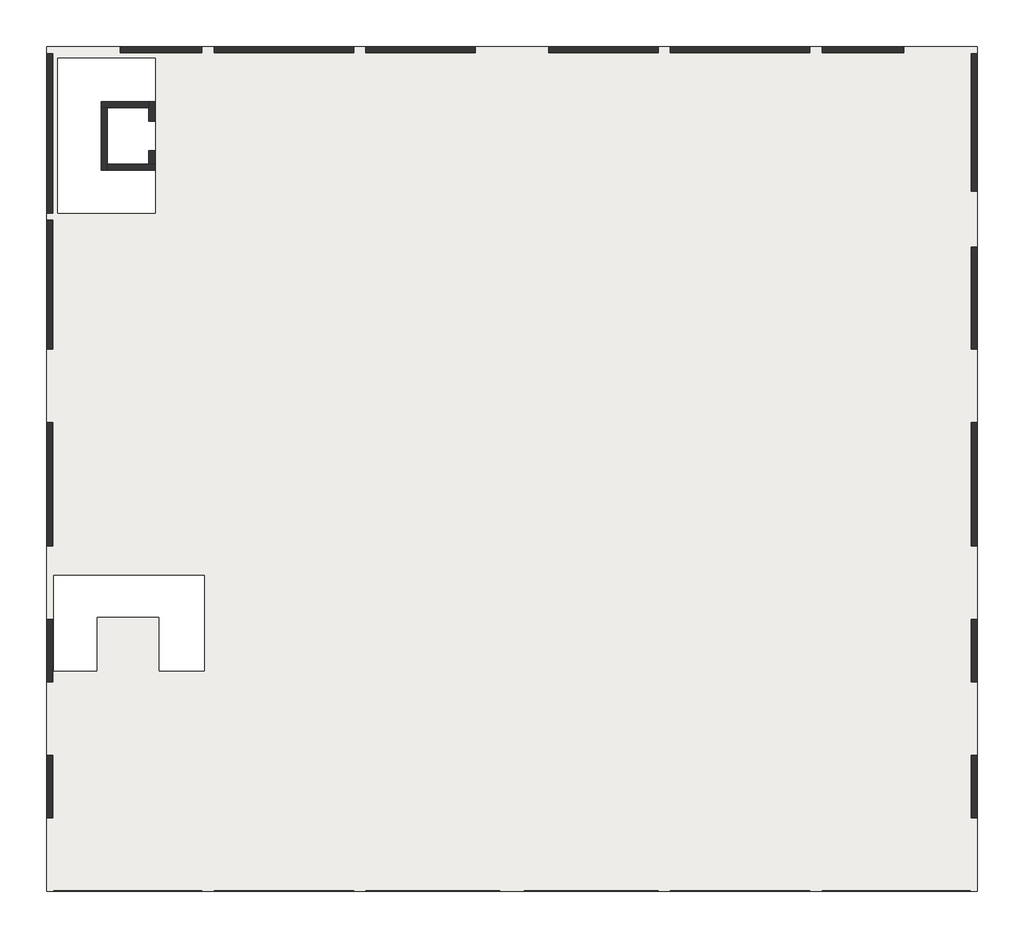
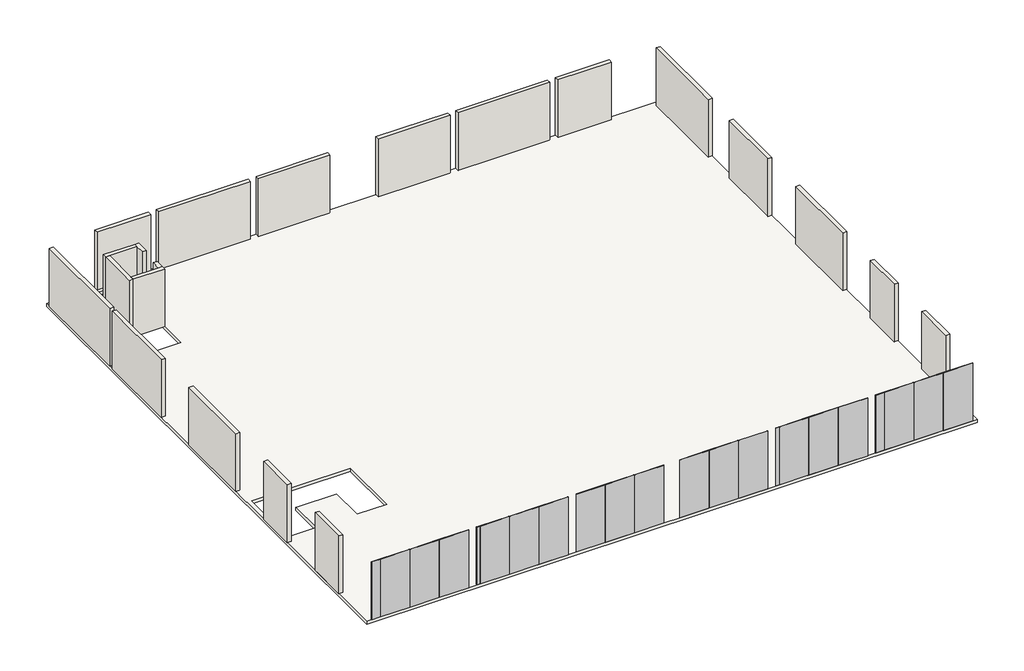
# One storey: 22 plates, 21 walls, 1 slab.
"""IFC4 building model written with IfcOpenShell, lengths in millimetres."""

import ifcopenshell
import ifcopenshell.guid

model = None  # the IFC model being written
_history = None  # IfcOwnerHistory: only IFC2X3 demands one
_inside = {}  # id of a spatial element -> (the spatial element, [elements in it])
_under = {}  # id of a project, library or spatial element -> (it, [spatial elements below it])
_declared = {}  # id of a project -> (the project, [libraries it declares])
_typed = {}  # id of a type object -> (the type object, [elements of that type])
_made_of = {}  # id of a material, layer set ... -> (it, [elements and type objects made of it])


def new_model(schema):
    """Start an empty IFC model of exactly this schema.

    Asked for "IFC4X3", IfcOpenShell would pick the latest addendum, in which some entities
    have other attributes; the version numbers below select the first issue.
    IFC2X3 requires an IfcOwnerHistory on every rooted entity: one is made here for all.
    """
    global model, _history
    if schema == "IFC4X3":
        model = ifcopenshell.file(schema_version=(4, 3, 0, 0))
    else:
        model = ifcopenshell.file(schema=schema)
    _inside.clear()
    _under.clear()
    _declared.clear()
    _typed.clear()
    _made_of.clear()
    _history = None
    if model.schema == "IFC2X3":
        org = make("IfcOrganization", Name="unknown")
        user = make(
            "IfcPersonAndOrganization",
            ThePerson=make("IfcPerson", FamilyName="unknown"),
            TheOrganization=org,
        )
        app = make(
            "IfcApplication",
            ApplicationDeveloper=org,
            Version="unknown",
            ApplicationFullName="unknown",
            ApplicationIdentifier="unknown",
        )
        _history = make(
            "IfcOwnerHistory",
            OwningUser=user,
            OwningApplication=app,
            ChangeAction="ADDED",
            CreationDate=0,
        )
    return model


def make(cls, **values):
    """One entity of the class cls with the attributes given. An attribute that is None is left unset."""
    return model.create_entity(
        cls, **{name: value for name, value in values.items() if value is not None}
    )


def rooted(cls, **values):
    """An entity with a GlobalId (a new one), such as an element, a storey or a relation."""
    return make(cls, GlobalId=ifcopenshell.guid.new(), OwnerHistory=_history, **values)


def si_unit(unit_type, name, prefix=None):
    """IfcSIUnit, for example si_unit("LENGTHUNIT", "METRE", prefix="MILLI")."""
    return make("IfcSIUnit", UnitType=unit_type, Prefix=prefix, Name=name)


def assignment(units):
    """IfcUnitAssignment: the units of a project."""
    return None if units is None else make("IfcUnitAssignment", Units=units)


def point(xyz):
    """IfcCartesianPoint."""
    return None if xyz is None else make("IfcCartesianPoint", Coordinates=xyz)


def direction(xyz):
    """IfcDirection."""
    return None if xyz is None else make("IfcDirection", DirectionRatios=xyz)


def frame(location, z_axis=None, x_axis=None):
    """IfcAxis2Placement3D, a coordinate frame: its origin and axes. An axis left out is left unset."""
    return make(
        "IfcAxis2Placement3D",
        Location=point(location),
        Axis=direction(z_axis),
        RefDirection=direction(x_axis),
    )


def origin():
    """The frame at (0, 0, 0) with its axes left unset."""
    return frame((0.0, 0.0, 0.0))


def origin_with_axes():
    """The frame at (0, 0, 0) with the z axis (0, 0, 1) and the x axis (1, 0, 0) written out."""
    return frame((0.0, 0.0, 0.0), z_axis=(0.0, 0.0, 1.0), x_axis=(1.0, 0.0, 0.0))


def place(relative_to, where):
    """IfcLocalPlacement: puts the frame where relative to a parent placement (None: the world)."""
    return make(
        "IfcLocalPlacement", PlacementRelTo=relative_to, RelativePlacement=where
    )


def context(
    kind, dimensions, precision=None, world=None, true_north=None, identifier=None
):
    """IfcGeometricRepresentationContext, for example the 3D "Model" context."""
    return make(
        "IfcGeometricRepresentationContext",
        ContextIdentifier=identifier,
        ContextType=kind,
        CoordinateSpaceDimension=dimensions,
        Precision=precision,
        WorldCoordinateSystem=world,
        TrueNorth=true_north,
    )


def project(units=None, contexts=None):
    """IfcProject with its units and contexts."""
    return rooted(
        "IfcProject",
        Name="project",
        RepresentationContexts=contexts,
        UnitsInContext=assignment(units),
    )


def spatial(cls, under=None, at=None, **own):
    """A site, building, storey or space (cls), placed at a placement, below another one or the project."""
    s = rooted(cls, ObjectPlacement=at, **own)
    if under is not None:
        _under.setdefault(under.id(), (under, []))[1].append(s)
    return s


def polyline(points):
    """IfcPolyline through the points."""
    return make("IfcPolyline", Points=[point(p) for p in points])


def outline(outer, holes=None, kind="AREA"):
    """IfcArbitraryClosedProfileDef: a profile drawn as a closed curve; with holes, ...WithVoids."""
    if holes is None:
        return make("IfcArbitraryClosedProfileDef", ProfileType=kind, OuterCurve=outer)
    return make(
        "IfcArbitraryProfileDefWithVoids",
        ProfileType=kind,
        OuterCurve=outer,
        InnerCurves=holes,
    )


def extrude(swept, where, along, depth):
    """IfcExtrudedAreaSolid: the profile swept, set in the frame where, extruded along a direction by depth."""
    return make(
        "IfcExtrudedAreaSolid",
        SweptArea=swept,
        Position=where,
        ExtrudedDirection=direction(along),
        Depth=depth,
    )


def faces_of(points, faces, orient=None, outer=None):
    """IfcFace entities. A face is a list of loops; a loop is a list of indices into points, from 0.

    orient and outer hold one flag for each loop. By default every Orientation is true, the
    first loop of a face is its IfcFaceOuterBound and the others are IfcFaceBound.
    """
    made = []
    for i, loops in enumerate(faces):
        bounds = []
        for j, loop in enumerate(loops):
            is_outer = j == 0 if outer is None else outer[i][j]
            bounds.append(
                make(
                    "IfcFaceOuterBound" if is_outer else "IfcFaceBound",
                    Bound=make("IfcPolyLoop", Polygon=[points[k] for k in loop]),
                    Orientation=True if orient is None else orient[i][j],
                )
            )
        made.append(make("IfcFace", Bounds=bounds))
    return made


def faceted_brep(points, faces, orient=None, outer=None, voids=None):
    """IfcFacetedBrep: a solid bounded by flat faces; with voids (closed shells), ...WithVoids."""
    shared = [point(p) for p in points]
    hull = make("IfcClosedShell", CfsFaces=faces_of(shared, faces, orient, outer))
    if voids is None:
        return make("IfcFacetedBrep", Outer=hull)
    return make(
        "IfcFacetedBrepWithVoids",
        Outer=hull,
        Voids=[
            make(cls, CfsFaces=faces_of(shared, fs, o, b)) for cls, fs, o, b in voids
        ],
    )


def shape(context_of_items, identifier, shape_type, items):
    """IfcShapeRepresentation: the items that make up one representation, for example the "Body"."""
    return make(
        "IfcShapeRepresentation",
        ContextOfItems=context_of_items,
        RepresentationIdentifier=identifier,
        RepresentationType=shape_type,
        Items=items,
    )


def source(mapping_origin, context_of_items, identifier, shape_type, items):
    """IfcRepresentationMap: a shape defined once, which mapped items show again and again."""
    return make(
        "IfcRepresentationMap",
        MappingOrigin=mapping_origin,
        MappedRepresentation=shape(context_of_items, identifier, shape_type, items),
    )


def transform(
    local_origin,
    x_axis=None,
    y_axis=None,
    z_axis=None,
    scale=None,
    scale2=None,
    scale3=None,
    uniform=True,
):
    """IfcCartesianTransformationOperator3D, or its non-uniform kind. x_axis, y_axis, z_axis: its Axis1, 2, 3."""
    if uniform:
        return make(
            "IfcCartesianTransformationOperator3D",
            Axis1=direction(x_axis),
            Axis2=direction(y_axis),
            LocalOrigin=point(local_origin),
            Scale=scale,
            Axis3=direction(z_axis),
        )
    return make(
        "IfcCartesianTransformationOperator3DnonUniform",
        Axis1=direction(x_axis),
        Axis2=direction(y_axis),
        LocalOrigin=point(local_origin),
        Scale=scale,
        Axis3=direction(z_axis),
        Scale2=scale2,
        Scale3=scale3,
    )


def mapped(mapping_source, mapping_target):
    """IfcMappedItem: shows the shape of a source again, moved by a transform."""
    return make(
        "IfcMappedItem", MappingSource=mapping_source, MappingTarget=mapping_target
    )


def made_of(thing, what):
    """Note that an element or type object is made of a material, layer set ...; save() writes the relation."""
    if what is not None:
        _made_of.setdefault(what.id(), (what, []))[1].append(thing)
    return thing


def element(
    cls,
    number,
    at=None,
    inside=None,
    cuts=None,
    type_object=None,
    material=None,
    context=None,
    identifier="Body",
    shape_type=None,
    held_by="IfcProductDefinitionShape",
    body=None,
    shapes=None,
    **own,
):
    """One element of the class cls, such as IfcWall. Its Tag is "e" and its number.

    at: its placement. inside: the storey or other place that contains it. cuts: it is an
    opening in that element (IfcRelVoidsElement). A single representation is given by context,
    identifier, shape_type and body (its items); several are given by shapes. held_by: the class
    of the entity that holds the representations. save() writes the other relations.
    """
    e = rooted(cls, Tag="e%d" % number, ObjectPlacement=at, **own)
    if body is not None:
        shapes = [shape(context, identifier, shape_type, body)]
    if shapes is not None:
        e.Representation = make(held_by, Representations=shapes)
    if inside is not None:
        _inside.setdefault(inside.id(), (inside, []))[1].append(e)
    if cuts is not None:
        rooted(
            "IfcRelVoidsElement", RelatingBuildingElement=cuts, RelatedOpeningElement=e
        )
    if type_object is not None:
        _typed.setdefault(type_object.id(), (type_object, []))[1].append(e)
    return made_of(e, material)


def aggregate(whole, parts):
    """IfcRelAggregates: a whole, such as a stair, and the parts it consists of."""
    return rooted("IfcRelAggregates", RelatingObject=whole, RelatedObjects=parts)


def save(model, path):
    """Write the relations noted so far, then the file.

    IfcRelAggregates (storeys below a building ...), IfcRelContainedInSpatialStructure (elements
    in a storey), IfcRelDefinesByType, IfcRelAssociatesMaterial and IfcRelDeclares: one each for
    every whole, place, type object, material and project.
    """
    for whole, parts in _under.values():
        aggregate(whole, parts)
    for where, things in _inside.values():
        rooted(
            "IfcRelContainedInSpatialStructure",
            RelatedElements=things,
            RelatingStructure=where,
        )
    for kind, things in _typed.values():
        rooted("IfcRelDefinesByType", RelatedObjects=things, RelatingType=kind)
    for what, things in _made_of.values():
        rooted("IfcRelAssociatesMaterial", RelatedObjects=things, RelatingMaterial=what)
    for by, libraries in _declared.values():
        rooted("IfcRelDeclares", RelatingContext=by, RelatedDefinitions=libraries)
    model.write(path)


def system_panel_glazed_0b61e5af(model_context):
    return source(origin(), model_context, "Body", "SweptSolid", [
        extrude(outline(polyline([(915.0000002, 24.5), (-915.0000002, 24.5), (-915.0000002, 49.5), (915.0000002, 49.5), (915.0000002, 24.5)])), origin_with_axes(), (0.0, 0.0, 1.0), 3800.0),
    ])


def system_panel_glazed_e3bcbcf3(model_context):
    return source(origin(), model_context, "Body", "SweptSolid", [
        extrude(outline(polyline([(274.9999998, 24.5), (-274.9999998, 24.5), (-274.9999998, 49.5), (274.9999998, 49.5), (274.9999998, 24.5)])), origin_with_axes(), (0.0, 0.0, 1.0), 3800.0),
    ])


def system_panel_glazed_31375f6b(model_context):
    return source(origin(), model_context, "Body", "SweptSolid", [
        extrude(outline(polyline([(104.9999998, 24.5), (-104.9999998, 24.5), (-104.9999998, 49.5), (104.9999998, 49.5), (104.9999998, 24.5)])), origin_with_axes(), (0.0, 0.0, 1.0), 3800.0),
    ])


def system_panel_glazed_aacaf49b(model_context):
    return source(origin(), model_context, "Body", "SweptSolid", [
        extrude(outline(polyline([(904.9999998, 24.5), (-904.9999998, 24.5), (-904.9999998, 49.5), (904.9999998, 49.5), (904.9999998, 24.5)])), origin_with_axes(), (0.0, 0.0, 1.0), 3800.0),
    ])


def system_panel_glazed_e1325fc6(model_context):
    return source(origin(), model_context, "Body", "SweptSolid", [
        extrude(outline(polyline([(894.9999998, 24.5), (-894.9999998, 24.5), (-894.9999998, 49.5), (894.9999998, 49.5), (894.9999998, 24.5)])), origin_with_axes(), (0.0, 0.0, 1.0), 3800.0),
    ])


model = new_model("IFC4")

# Units and contexts
model_context = context("Model", 3, world=origin())
ifc_project = project(units=[si_unit("LENGTHUNIT", "METRE", prefix="MILLI")], contexts=[model_context])

# Site, building, storey
site = spatial("IfcSite", under=ifc_project)
building = spatial("IfcBuilding", under=site)
storey = spatial("IfcBuildingStorey", under=building, Name="Perdhesa", Elevation=0.0)

# Plates
placement = place(None, origin())
system_panel_glazed_shape = system_panel_glazed_0b61e5af(model_context)
element("IfcPlate", 1, ObjectType="System Panel : Glazed", at=placement, inside=storey, context=model_context, shape_type="MappedRepresentation", body=[
    mapped(system_panel_glazed_shape, transform((18910.5819109, -16669.9481037, 0.0), x_axis=(-1.0, 0.0, 0.0), y_axis=(0.0, -1.0, 0.0), z_axis=(0.0, 0.0, 1.0))),
])
element("IfcPlate", 2, ObjectType="System Panel : Glazed", at=placement, inside=storey, context=model_context, shape_type="MappedRepresentation", body=[
    mapped(system_panel_glazed_shape, transform((17080.5819107, -16669.9481037, 0.0), x_axis=(-1.0, 0.0, 0.0), y_axis=(0.0, -1.0, 0.0), z_axis=(0.0, 0.0, 1.0))),
])
element("IfcPlate", 3, ObjectType="System Panel : Glazed", at=placement, inside=storey, context=model_context, shape_type="MappedRepresentation", body=[
    mapped(system_panel_glazed_shape, transform((15250.5819107, -16669.9481037, 0.0), x_axis=(-1.0, 0.0, 0.0), y_axis=(0.0, -1.0, 0.0), z_axis=(0.0, 0.0, 1.0))),
])
element("IfcPlate", 4, ObjectType="System Panel : Glazed", at=placement, inside=storey, context=model_context, shape_type="MappedRepresentation", body=[
    mapped(system_panel_glazed_shape, transform((12370.5819109, -16669.9481037, 0.0), x_axis=(-1.0, 0.0, 0.0), y_axis=(0.0, -1.0, 0.0), z_axis=(0.0, 0.0, 1.0))),
])
element("IfcPlate", 5, ObjectType="System Panel : Glazed", at=placement, inside=storey, context=model_context, shape_type="MappedRepresentation", body=[
    mapped(system_panel_glazed_shape, transform((10540.5819107, -16669.9481037, 0.0), x_axis=(-1.0, 0.0, 0.0), y_axis=(0.0, -1.0, 0.0), z_axis=(0.0, 0.0, 1.0))),
])
element("IfcPlate", 6, ObjectType="System Panel : Glazed", at=placement, inside=storey, context=model_context, shape_type="MappedRepresentation", body=[
    mapped(system_panel_glazed_shape, transform((8710.5819107, -16669.9481037, 0.0), x_axis=(-1.0, 0.0, 0.0), y_axis=(0.0, -1.0, 0.0), z_axis=(0.0, 0.0, 1.0))),
])
element("IfcPlate", 7, ObjectType="System Panel : Glazed", at=placement, inside=storey, context=model_context, shape_type="MappedRepresentation", body=[
    mapped(system_panel_glazed_shape, transform((6170.5819109, -16669.9481037, 0.0), x_axis=(-1.0, 0.0, 0.0), y_axis=(0.0, -1.0, 0.0), z_axis=(0.0, 0.0, 1.0))),
])
element("IfcPlate", 8, ObjectType="System Panel : Glazed", at=placement, inside=storey, context=model_context, shape_type="MappedRepresentation", body=[
    mapped(system_panel_glazed_shape, transform((4340.5819107, -16669.9481037, 0.0), x_axis=(-1.0, 0.0, 0.0), y_axis=(0.0, -1.0, 0.0), z_axis=(0.0, 0.0, 1.0))),
])
element("IfcPlate", 9, ObjectType="System Panel : Glazed", at=placement, inside=storey, context=model_context, shape_type="MappedRepresentation", body=[
    mapped(system_panel_glazed_shape, transform((-299.4180891, -16669.9481037, 0.0), x_axis=(-1.0, 0.0, 0.0), y_axis=(0.0, -1.0, 0.0), z_axis=(0.0, 0.0, 1.0))),
])
element("IfcPlate", 10, ObjectType="System Panel : Glazed", at=placement, inside=storey, context=model_context, shape_type="MappedRepresentation", body=[
    mapped(system_panel_glazed_shape, transform((-2129.4180893, -16669.9481037, 0.0), x_axis=(-1.0, 0.0, 0.0), y_axis=(0.0, -1.0, 0.0), z_axis=(0.0, 0.0, 1.0))),
])
element("IfcPlate", 11, ObjectType="System Panel : Glazed", at=placement, inside=storey, context=model_context, shape_type="MappedRepresentation", body=[
    mapped(system_panel_glazed_shape, transform((-6249.4180891, -16669.9481037, 0.0), x_axis=(-1.0, 0.0, 0.0), y_axis=(0.0, -1.0, 0.0), z_axis=(0.0, 0.0, 1.0))),
])
element("IfcPlate", 12, ObjectType="System Panel : Glazed", at=placement, inside=storey, context=model_context, shape_type="MappedRepresentation", body=[
    mapped(system_panel_glazed_shape, transform((-8079.4180893, -16669.9481037, 0.0), x_axis=(-1.0, 0.0, 0.0), y_axis=(0.0, -1.0, 0.0), z_axis=(0.0, 0.0, 1.0))),
])
element("IfcPlate", 13, ObjectType="System Panel : Glazed", at=placement, inside=storey, context=model_context, shape_type="MappedRepresentation", body=[
    mapped(system_panel_glazed_shape, transform((-9909.4180893, -16669.9481037, 0.0), x_axis=(-1.0, 0.0, 0.0), y_axis=(0.0, -1.0, 0.0), z_axis=(0.0, 0.0, 1.0))),
])
element("IfcPlate", 14, ObjectType="System Panel : Glazed", at=placement, inside=storey, context=model_context, shape_type="MappedRepresentation", body=[
    mapped(system_panel_glazed_shape, transform((-12449.4180891, -16669.9481037, 0.0), x_axis=(-1.0, 0.0, 0.0), y_axis=(0.0, -1.0, 0.0), z_axis=(0.0, 0.0, 1.0))),
])
element("IfcPlate", 15, ObjectType="System Panel : Glazed", at=placement, inside=storey, context=model_context, shape_type="MappedRepresentation", body=[
    mapped(system_panel_glazed_shape, transform((-14279.4180893, -16669.9481037, 0.0), x_axis=(-1.0, 0.0, 0.0), y_axis=(0.0, -1.0, 0.0), z_axis=(0.0, 0.0, 1.0))),
])
element("IfcPlate", 16, ObjectType="System Panel : Glazed", at=placement, inside=storey, context=model_context, shape_type="MappedRepresentation", body=[
    mapped(system_panel_glazed_shape, transform((-16109.4180893, -16669.9481037, 0.0), x_axis=(-1.0, 0.0, 0.0), y_axis=(0.0, -1.0, 0.0), z_axis=(0.0, 0.0, 1.0))),
])
system_panel_glazed_2_shape = system_panel_glazed_e3bcbcf3(model_context)
element("IfcPlate", 17, ObjectType="System Panel : Glazed", at=placement, inside=storey, context=model_context, shape_type="MappedRepresentation", body=[
    mapped(system_panel_glazed_2_shape, transform((14060.5819109, -16669.9481037, 0.0), x_axis=(-1.0, 0.0, 0.0), y_axis=(0.0, -1.0, 0.0), z_axis=(0.0, 0.0, 1.0))),
])
element("IfcPlate", 18, ObjectType="System Panel : Glazed", at=placement, inside=storey, context=model_context, shape_type="MappedRepresentation", body=[
    mapped(system_panel_glazed_2_shape, transform((-17299.4180891, -16669.9481037, 0.0), x_axis=(-1.0, 0.0, 0.0), y_axis=(0.0, -1.0, 0.0), z_axis=(0.0, 0.0, 1.0))),
])
system_panel_glazed_3_shape = system_panel_glazed_31375f6b(model_context)
element("IfcPlate", 19, ObjectType="System Panel : Glazed", at=placement, inside=storey, context=model_context, shape_type="MappedRepresentation", body=[
    mapped(system_panel_glazed_3_shape, transform((7690.5819109, -16669.9481037, 0.0), x_axis=(-1.0, 0.0, 0.0), y_axis=(0.0, -1.0, 0.0), z_axis=(0.0, 0.0, 1.0))),
])
element("IfcPlate", 20, ObjectType="System Panel : Glazed", at=placement, inside=storey, context=model_context, shape_type="MappedRepresentation", body=[
    mapped(system_panel_glazed_3_shape, transform((-10929.4180891, -16669.9481037, 0.0), x_axis=(-1.0, 0.0, 0.0), y_axis=(0.0, -1.0, 0.0), z_axis=(0.0, 0.0, 1.0))),
])
system_panel_glazed_4_shape = system_panel_glazed_aacaf49b(model_context)
element("IfcPlate", 21, ObjectType="System Panel : Glazed", at=placement, inside=storey, context=model_context, shape_type="MappedRepresentation", body=[
    mapped(system_panel_glazed_4_shape, transform((2520.5819109, -16669.9481037, 0.0), x_axis=(-1.0, 0.0, 0.0), y_axis=(0.0, -1.0, 0.0), z_axis=(0.0, 0.0, 1.0))),
])
system_panel_glazed_5_shape = system_panel_glazed_e1325fc6(model_context)
element("IfcPlate", 22, ObjectType="System Panel : Glazed", at=placement, inside=storey, context=model_context, shape_type="MappedRepresentation", body=[
    mapped(system_panel_glazed_5_shape, transform((-3939.4180891, -16669.9481037, 0.0), x_axis=(-1.0, 0.0, 0.0), y_axis=(0.0, -1.0, 0.0), z_axis=(0.0, 0.0, 1.0))),
])

# Slab
element("IfcSlab", 23, ObjectType="Generic 20", at=placement, inside=storey, context=model_context, shape_type="SweptSolid", body=[
    extrude(outline(polyline([(20125.581911, 17780.6768963), (20125.581911, -16719.3231037), (-17874.418089, -16719.3231037), (-17874.418089, 17780.6768963), (20125.581911, 17780.6768963)]), holes=[polyline([(-17424.418089, 17310.6768963), (-17424.418089, 10980.6768963), (-13444.418089, 10980.6768963), (-13444.418089, 17310.6768963), (-17424.418089, 17310.6768963)]), polyline([(-15825.6814495, -5518.0731037), (-13265.2814495, -5518.0731037), (-13265.2814495, -7718.0731037), (-11435.2814495, -7718.0731037), (-11435.2814495, -3818.0731037), (-17574.418089, -3818.0731037), (-17574.418089, -7718.0731037), (-15825.6814495, -7718.0731037), (-15825.6814495, -5518.0731037)])]), frame((0.0, 0.0, -200.0), z_axis=(0.0, 0.0, 1.0), x_axis=(1.0, 0.0, 0.0)), (0.0, 0.0, 1.0), 200.0),
])

# Walls
element("IfcWall", 24, ObjectType="lifti", at=placement, inside=storey, context=model_context, shape_type="Brep", body=[
    faceted_brep([(-15644.418089, 15280.6768963, 0.0), (-15394.418089, 15280.6768963, 0.0), (-13694.418089, 15280.6768963, 0.0), (-13694.418089, 15280.6768963, 3800.0), (-15394.418089, 15280.6768963, 3800.0), (-15644.418089, 15280.6768963, 3800.0), (-15644.418089, 15530.6768963, 0.0), (-15644.418089, 15530.6768963, 3800.0), (-13694.418089, 15530.6768963, 3800.0), (-13694.418089, 15530.6768963, 0.0)], [[[0, 1, 2, 3, 4, 5]], [[6, 7, 8, 9]], [[2, 1, 0, 6, 9]], [[5, 4, 3, 8, 7]], [[0, 5, 7, 6]], [[3, 2, 9, 8]]]),
])
element("IfcWall", 25, ObjectType="lifti", at=placement, inside=storey, context=model_context, shape_type="Brep", body=[
    faceted_brep([(-15394.418089, 12730.6768963, 0.0), (-15394.418089, 12980.6768963, 0.0), (-15394.418089, 15280.6768963, 0.0), (-15394.418089, 15280.6768963, 3800.0), (-15394.418089, 12980.6768963, 3800.0), (-15394.418089, 12730.6768963, 3800.0), (-15644.418089, 12730.6768963, 0.0), (-15644.418089, 12730.6768963, 3800.0), (-15644.418089, 15280.6768963, 3800.0), (-15644.418089, 15280.6768963, 0.0)], [[[0, 1, 2, 3, 4, 5]], [[6, 7, 8, 9]], [[2, 1, 0, 6, 9]], [[5, 4, 3, 8, 7]], [[0, 5, 7, 6]], [[3, 2, 9, 8]]]),
])
element("IfcWall", 26, ObjectType="lifti", at=placement, inside=storey, context=model_context, shape_type="Brep", body=[
    faceted_brep([(-13444.418089, 12980.6768963, 0.0), (-13694.418089, 12980.6768963, 0.0), (-15394.418089, 12980.6768963, 0.0), (-15394.418089, 12980.6768963, 3800.0), (-13694.418089, 12980.6768963, 3800.0), (-13444.418089, 12980.6768963, 3800.0), (-13444.418089, 12730.6768963, 0.0), (-13444.418089, 12730.6768963, 3800.0), (-15394.418089, 12730.6768963, 3800.0), (-15394.418089, 12730.6768963, 0.0)], [[[0, 1, 2, 3, 4, 5]], [[6, 7, 8, 9]], [[2, 1, 0, 6, 9]], [[5, 4, 3, 8, 7]], [[0, 5, 7, 6]], [[3, 2, 9, 8]]]),
])
element("IfcWall", 27, ObjectType="lifti", at=placement, inside=storey, context=model_context, shape_type="Brep", body=[
    faceted_brep([(-13694.418089, 15530.6768963, 0.0), (-13694.418089, 15280.6768963, 0.0), (-13694.418089, 14730.6768963, 0.0), (-13694.418089, 14730.6768963, 3800.0), (-13694.418089, 15280.6768963, 3800.0), (-13694.418089, 15530.6768963, 3800.0), (-13444.418089, 15530.6768963, 0.0), (-13444.418089, 15530.6768963, 3800.0), (-13444.418089, 14730.6768963, 3800.0), (-13444.418089, 14730.6768963, 0.0)], [[[0, 1, 2, 3, 4, 5]], [[6, 7, 8, 9]], [[2, 1, 0, 6, 9]], [[3, 2, 9, 8]], [[5, 4, 3, 8, 7]], [[0, 5, 7, 6]]]),
])
element("IfcWall", 28, ObjectType="lifti", at=placement, inside=storey, context=model_context, shape_type="SweptSolid", body=[
    extrude(outline(polyline([(-13694.418089, 12980.6768963), (-13694.418089, 13530.6768963), (-13444.418089, 13530.6768963), (-13444.418089, 12980.6768963), (-13694.418089, 12980.6768963)])), origin_with_axes(), (0.0, 0.0, 1.0), 3800.0),
])
element("IfcWall", 29, ObjectType="Generic - 250", at=placement, inside=storey, context=model_context, shape_type="SweptSolid", body=[
    extrude(outline(polyline([(-17874.418089, 10980.6768963), (-17874.418089, 17480.6768963), (-17624.418089, 17480.6768963), (-17624.418089, 10980.6768963), (-17874.418089, 10980.6768963)])), origin_with_axes(), (0.0, 0.0, 1.0), 3800.0),
])
element("IfcWall", 30, ObjectType="Generic - 250", at=placement, inside=storey, context=model_context, shape_type="SweptSolid", body=[
    extrude(outline(polyline([(-11534.418089, 17530.6768963), (-14874.418089, 17530.6768963), (-14874.418089, 17780.6768963), (-11534.418089, 17780.6768963), (-11534.418089, 17530.6768963)])), origin_with_axes(), (0.0, 0.0, 1.0), 3800.0),
])
element("IfcWall", 31, ObjectType="Generic - 250", at=placement, inside=storey, context=model_context, shape_type="SweptSolid", body=[
    extrude(outline(polyline([(-5334.418089, 17530.6768963), (-11034.418089, 17530.6768963), (-11034.418089, 17780.6768963), (-5334.418089, 17780.6768963), (-5334.418089, 17530.6768963)])), origin_with_axes(), (0.0, 0.0, 1.0), 3800.0),
])
element("IfcWall", 32, ObjectType="Generic - 250", at=placement, inside=storey, context=model_context, shape_type="SweptSolid", body=[
    extrude(outline(polyline([(-384.418089, 17530.6768963), (-4834.418089, 17530.6768963), (-4834.418089, 17780.6768963), (-384.418089, 17780.6768963), (-384.418089, 17530.6768963)])), origin_with_axes(), (0.0, 0.0, 1.0), 3800.0),
])
element("IfcWall", 33, ObjectType="Generic - 250", at=placement, inside=storey, context=model_context, shape_type="SweptSolid", body=[
    extrude(outline(polyline([(7085.581911, 17530.6768963), (2615.581911, 17530.6768963), (2615.581911, 17780.6768963), (7085.581911, 17780.6768963), (7085.581911, 17530.6768963)])), origin_with_axes(), (0.0, 0.0, 1.0), 3800.0),
])
element("IfcWall", 34, ObjectType="Generic - 250", at=placement, inside=storey, context=model_context, shape_type="SweptSolid", body=[
    extrude(outline(polyline([(13285.581911, 17530.6768963), (7585.581911, 17530.6768963), (7585.581911, 17780.6768963), (13285.581911, 17780.6768963), (13285.581911, 17530.6768963)])), origin_with_axes(), (0.0, 0.0, 1.0), 3800.0),
])
element("IfcWall", 35, ObjectType="Generic - 250", at=placement, inside=storey, context=model_context, shape_type="SweptSolid", body=[
    extrude(outline(polyline([(17125.581911, 17530.6768963), (13785.581911, 17530.6768963), (13785.581911, 17780.6768963), (17125.581911, 17780.6768963), (17125.581911, 17530.6768963)])), origin_with_axes(), (0.0, 0.0, 1.0), 3800.0),
])
element("IfcWall", 36, ObjectType="Generic - 250", at=placement, inside=storey, context=model_context, shape_type="SweptSolid", body=[
    extrude(outline(polyline([(19875.581911, 11880.6768963), (19875.581911, 17480.6768963), (20125.581911, 17480.6768963), (20125.581911, 11880.6768963), (19875.581911, 11880.6768963)])), origin_with_axes(), (0.0, 0.0, 1.0), 3800.0),
])
element("IfcWall", 37, ObjectType="Generic - 250", at=placement, inside=storey, context=model_context, shape_type="SweptSolid", body=[
    extrude(outline(polyline([(19875.581911, 5430.6768963), (19875.581911, 9580.6768963), (20125.581911, 9580.6768963), (20125.581911, 5430.6768963), (19875.581911, 5430.6768963)])), origin_with_axes(), (0.0, 0.0, 1.0), 3800.0),
])
element("IfcWall", 38, ObjectType="Generic - 250", at=placement, inside=storey, context=model_context, shape_type="SweptSolid", body=[
    extrude(outline(polyline([(19875.581911, -2619.3231037), (19875.581911, 2430.6768963), (20125.581911, 2430.6768963), (20125.581911, -2619.3231037), (19875.581911, -2619.3231037)])), origin_with_axes(), (0.0, 0.0, 1.0), 3800.0),
])
element("IfcWall", 39, ObjectType="Generic - 250", at=placement, inside=storey, context=model_context, shape_type="SweptSolid", body=[
    extrude(outline(polyline([(19875.581911, -8169.3231037), (19875.581911, -5619.3231037), (20125.581911, -5619.3231037), (20125.581911, -8169.3231037), (19875.581911, -8169.3231037)])), origin_with_axes(), (0.0, 0.0, 1.0), 3800.0),
])
element("IfcWall", 40, ObjectType="Generic - 250", at=placement, inside=storey, context=model_context, shape_type="SweptSolid", body=[
    extrude(outline(polyline([(19875.581911, -13719.3231037), (19875.581911, -11169.3231037), (20125.581911, -11169.3231037), (20125.581911, -13719.3231037), (19875.581911, -13719.3231037)])), origin_with_axes(), (0.0, 0.0, 1.0), 3800.0),
])
element("IfcWall", 41, ObjectType="Generic - 250", at=placement, inside=storey, context=model_context, shape_type="SweptSolid", body=[
    extrude(outline(polyline([(-17624.418089, -11169.3231037), (-17624.418089, -13719.3231037), (-17874.418089, -13719.3231037), (-17874.418089, -11169.3231037), (-17624.418089, -11169.3231037)])), origin_with_axes(), (0.0, 0.0, 1.0), 3800.0),
])
element("IfcWall", 42, ObjectType="Generic - 250", at=placement, inside=storey, context=model_context, shape_type="SweptSolid", body=[
    extrude(outline(polyline([(-17624.418089, -5619.3231037), (-17624.418089, -8169.3231037), (-17874.418089, -8169.3231037), (-17874.418089, -5619.3231037), (-17624.418089, -5619.3231037)])), origin_with_axes(), (0.0, 0.0, 1.0), 3800.0),
])
element("IfcWall", 43, ObjectType="Generic - 250", at=placement, inside=storey, context=model_context, shape_type="SweptSolid", body=[
    extrude(outline(polyline([(-17624.418089, 2430.6768963), (-17624.418089, -2619.3231037), (-17874.418089, -2619.3231037), (-17874.418089, 2430.6768963), (-17624.418089, 2430.6768963)])), origin_with_axes(), (0.0, 0.0, 1.0), 3800.0),
])
element("IfcWall", 44, ObjectType="Generic - 250", at=placement, inside=storey, context=model_context, shape_type="SweptSolid", body=[
    extrude(outline(polyline([(-17624.418089, 10680.6768963), (-17624.418089, 5430.6768963), (-17874.418089, 5430.6768963), (-17874.418089, 10680.6768963), (-17624.418089, 10680.6768963)])), origin_with_axes(), (0.0, 0.0, 1.0), 3800.0),
])

save(model, "model.ifc")

# Revit data of these elements
# Type "System Panel : Glazed"
#   Construction Type Id = "GSP4R"
#   Analytic Construction = "1/8 in Pilkington single glazing"
#   Visual Light Transmittance = 0.9
#   Solar Heat Gain Coefficient = 0.86
#   Heat Transfer Coefficient (U) = 6.7069 W/(m²·K)
#   Define Thermal Properties by = 1
# Type "Generic 20"
#   Function = 0
#   Layers, outside or top first: 20 cm no material (function 1)
# Type "lifti"
#   Layers, outside or top first: 25 cm "Concrete, C20/25" (function 1)
# Type "Generic - 250"
#   Layers, outside or top first: 25 cm no material (function 1)
# Elements 1, 2, 3, 4, 5, 6, 7, 8, 9, 10, 11, 12, 13, 14, 15, 16, 17, 18, 19, 20, 21, 22 (IfcPlate, "System Panel : Glazed")
#   Phase Created = New Construction
#   Materials on its faces: "Glass"
# Element 23 (IfcSlab, "Generic 20")
#   Height Offset From Level = 0 cm
#   Phase Created = New Construction
#   Materials on its faces: "Default Floor"
# Elements 24, 25, 26, 27, 28 (IfcWall, "lifti")
#   Top Offset = -20 cm
#   Base Offset = 0 cm
#   wall height = 380 cm
#   Phase Created = New Construction
#   Base Constraint = Perdhesa
#   Top Constraint = Kati1
#   Materials on its faces: "Concrete, C20/25"
# Elements 29, 30, 31, 32, 33, 34, 35, 36, 37, 38, 39, 40, 41, 42, 43, 44 (IfcWall, "Generic - 250")
#   Top Offset = -20 cm
#   Base Offset = 0 cm
#   wall height = 380 cm
#   Phase Created = New Construction
#   Base Constraint = Perdhesa
#   Top Constraint = Kati1
#   Materials on its faces: "Default Wall"
# Materials
#   "Concrete, C20/25": class "Metal", colour RGB 120 120 120, transparency 0, Description = "Eurocode concrete, 20MPa", Cost = 0
#   "Glass": class "Glass", colour RGB 0 128 192, transparency 0.9, Description = "Soda Lime Glass", Cost = 0
#   "Default Floor": class "Miscellaneous", colour RGB 127 127 127, transparency 0, Cost = 0
#   "Default Wall": class "Miscellaneous", colour RGB 128 128 128, transparency 0, Cost = 0
